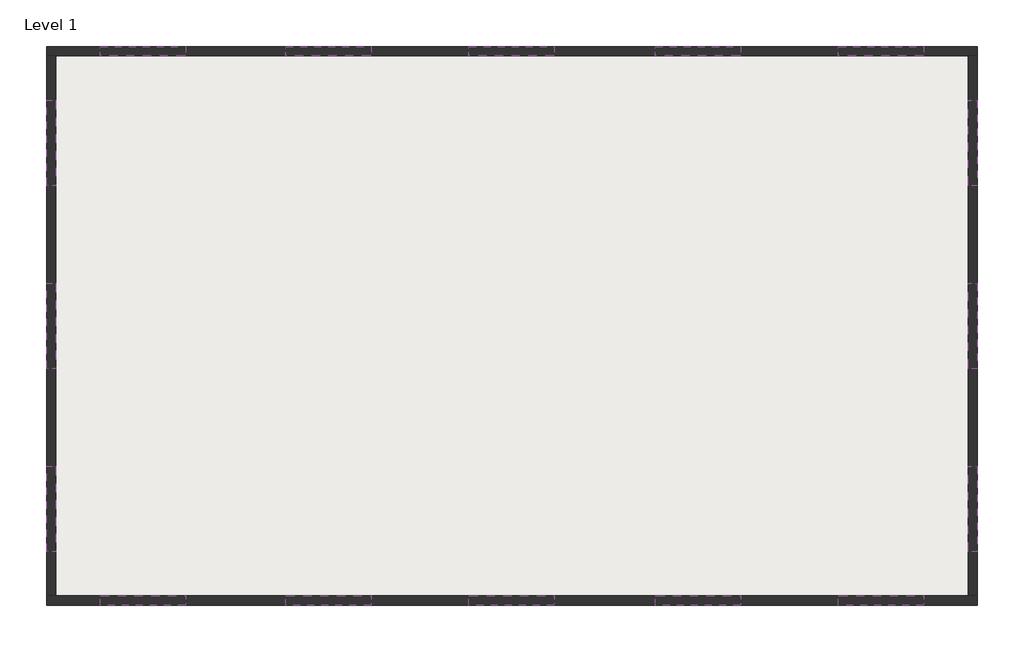
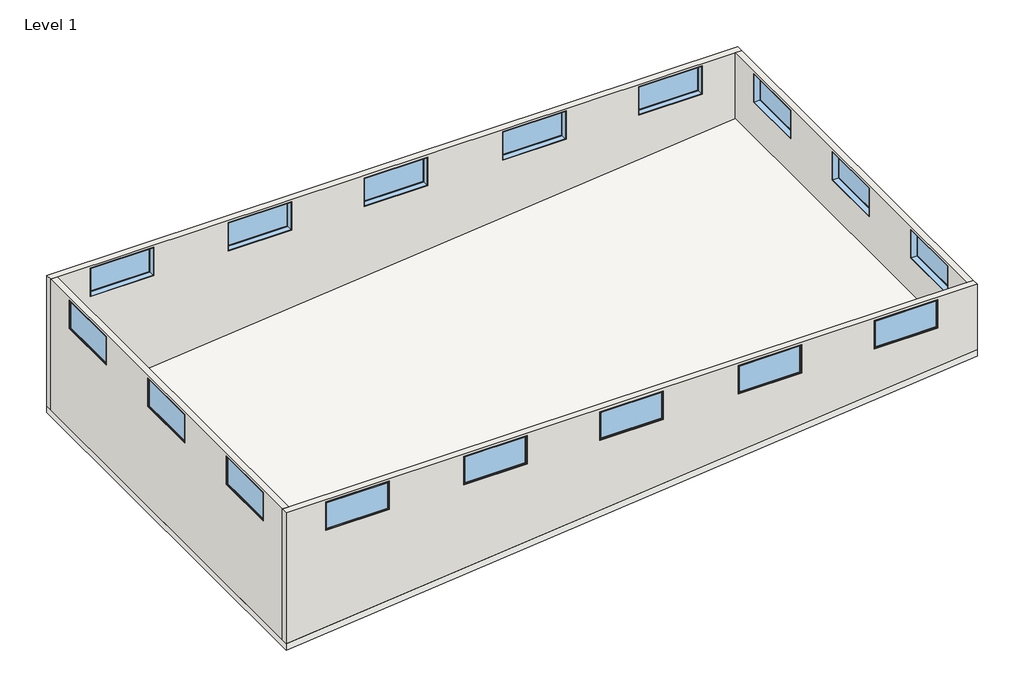
# One storey: 16 windows, 4 walls, 1 slab.
"""IFC4 building model written with IfcOpenShell, lengths in millimetres."""

import ifcopenshell
import ifcopenshell.guid

model = None  # the IFC model being written
_history = None  # IfcOwnerHistory: only IFC2X3 demands one
_inside = {}  # id of a spatial element -> (the spatial element, [elements in it])
_under = {}  # id of a project, library or spatial element -> (it, [spatial elements below it])
_declared = {}  # id of a project -> (the project, [libraries it declares])
_typed = {}  # id of a type object -> (the type object, [elements of that type])
_made_of = {}  # id of a material, layer set ... -> (it, [elements and type objects made of it])


def new_model(schema):
    """Start an empty IFC model of exactly this schema.

    Asked for "IFC4X3", IfcOpenShell would pick the latest addendum, in which some entities
    have other attributes; the version numbers below select the first issue.
    IFC2X3 requires an IfcOwnerHistory on every rooted entity: one is made here for all.
    """
    global model, _history
    if schema == "IFC4X3":
        model = ifcopenshell.file(schema_version=(4, 3, 0, 0))
    else:
        model = ifcopenshell.file(schema=schema)
    _inside.clear()
    _under.clear()
    _declared.clear()
    _typed.clear()
    _made_of.clear()
    _history = None
    if model.schema == "IFC2X3":
        org = make("IfcOrganization", Name="unknown")
        user = make(
            "IfcPersonAndOrganization",
            ThePerson=make("IfcPerson", FamilyName="unknown"),
            TheOrganization=org,
        )
        app = make(
            "IfcApplication",
            ApplicationDeveloper=org,
            Version="unknown",
            ApplicationFullName="unknown",
            ApplicationIdentifier="unknown",
        )
        _history = make(
            "IfcOwnerHistory",
            OwningUser=user,
            OwningApplication=app,
            ChangeAction="ADDED",
            CreationDate=0,
        )
    return model


def make(cls, **values):
    """One entity of the class cls with the attributes given. An attribute that is None is left unset."""
    return model.create_entity(
        cls, **{name: value for name, value in values.items() if value is not None}
    )


def rooted(cls, **values):
    """An entity with a GlobalId (a new one), such as an element, a storey or a relation."""
    return make(cls, GlobalId=ifcopenshell.guid.new(), OwnerHistory=_history, **values)


def si_unit(unit_type, name, prefix=None):
    """IfcSIUnit, for example si_unit("LENGTHUNIT", "METRE", prefix="MILLI")."""
    return make("IfcSIUnit", UnitType=unit_type, Prefix=prefix, Name=name)


def assignment(units):
    """IfcUnitAssignment: the units of a project."""
    return None if units is None else make("IfcUnitAssignment", Units=units)


def point(xyz):
    """IfcCartesianPoint."""
    return None if xyz is None else make("IfcCartesianPoint", Coordinates=xyz)


def direction(xyz):
    """IfcDirection."""
    return None if xyz is None else make("IfcDirection", DirectionRatios=xyz)


def frame(location, z_axis=None, x_axis=None):
    """IfcAxis2Placement3D, a coordinate frame: its origin and axes. An axis left out is left unset."""
    return make(
        "IfcAxis2Placement3D",
        Location=point(location),
        Axis=direction(z_axis),
        RefDirection=direction(x_axis),
    )


def origin():
    """The frame at (0, 0, 0) with its axes left unset."""
    return frame((0.0, 0.0, 0.0))


def place(relative_to, where):
    """IfcLocalPlacement: puts the frame where relative to a parent placement (None: the world)."""
    return make(
        "IfcLocalPlacement", PlacementRelTo=relative_to, RelativePlacement=where
    )


def context(
    kind, dimensions, precision=None, world=None, true_north=None, identifier=None
):
    """IfcGeometricRepresentationContext, for example the 3D "Model" context."""
    return make(
        "IfcGeometricRepresentationContext",
        ContextIdentifier=identifier,
        ContextType=kind,
        CoordinateSpaceDimension=dimensions,
        Precision=precision,
        WorldCoordinateSystem=world,
        TrueNorth=true_north,
    )


def project(units=None, contexts=None):
    """IfcProject with its units and contexts."""
    return rooted(
        "IfcProject",
        Name="project",
        RepresentationContexts=contexts,
        UnitsInContext=assignment(units),
    )


def spatial(cls, under=None, at=None, **own):
    """A site, building, storey or space (cls), placed at a placement, below another one or the project."""
    s = rooted(cls, ObjectPlacement=at, **own)
    if under is not None:
        _under.setdefault(under.id(), (under, []))[1].append(s)
    return s


def polyline(points):
    """IfcPolyline through the points."""
    return make("IfcPolyline", Points=[point(p) for p in points])


def outline(outer, holes=None, kind="AREA"):
    """IfcArbitraryClosedProfileDef: a profile drawn as a closed curve; with holes, ...WithVoids."""
    if holes is None:
        return make("IfcArbitraryClosedProfileDef", ProfileType=kind, OuterCurve=outer)
    return make(
        "IfcArbitraryProfileDefWithVoids",
        ProfileType=kind,
        OuterCurve=outer,
        InnerCurves=holes,
    )


def extrude(swept, where, along, depth):
    """IfcExtrudedAreaSolid: the profile swept, set in the frame where, extruded along a direction by depth."""
    return make(
        "IfcExtrudedAreaSolid",
        SweptArea=swept,
        Position=where,
        ExtrudedDirection=direction(along),
        Depth=depth,
    )


def faces_of(points, faces, orient=None, outer=None):
    """IfcFace entities. A face is a list of loops; a loop is a list of indices into points, from 0.

    orient and outer hold one flag for each loop. By default every Orientation is true, the
    first loop of a face is its IfcFaceOuterBound and the others are IfcFaceBound.
    """
    made = []
    for i, loops in enumerate(faces):
        bounds = []
        for j, loop in enumerate(loops):
            is_outer = j == 0 if outer is None else outer[i][j]
            bounds.append(
                make(
                    "IfcFaceOuterBound" if is_outer else "IfcFaceBound",
                    Bound=make("IfcPolyLoop", Polygon=[points[k] for k in loop]),
                    Orientation=True if orient is None else orient[i][j],
                )
            )
        made.append(make("IfcFace", Bounds=bounds))
    return made


def faceted_brep(points, faces, orient=None, outer=None, voids=None):
    """IfcFacetedBrep: a solid bounded by flat faces; with voids (closed shells), ...WithVoids."""
    shared = [point(p) for p in points]
    hull = make("IfcClosedShell", CfsFaces=faces_of(shared, faces, orient, outer))
    if voids is None:
        return make("IfcFacetedBrep", Outer=hull)
    return make(
        "IfcFacetedBrepWithVoids",
        Outer=hull,
        Voids=[
            make(cls, CfsFaces=faces_of(shared, fs, o, b)) for cls, fs, o, b in voids
        ],
    )


def shape(context_of_items, identifier, shape_type, items):
    """IfcShapeRepresentation: the items that make up one representation, for example the "Body"."""
    return make(
        "IfcShapeRepresentation",
        ContextOfItems=context_of_items,
        RepresentationIdentifier=identifier,
        RepresentationType=shape_type,
        Items=items,
    )


def source(mapping_origin, context_of_items, identifier, shape_type, items):
    """IfcRepresentationMap: a shape defined once, which mapped items show again and again."""
    return make(
        "IfcRepresentationMap",
        MappingOrigin=mapping_origin,
        MappedRepresentation=shape(context_of_items, identifier, shape_type, items),
    )


def transform(
    local_origin,
    x_axis=None,
    y_axis=None,
    z_axis=None,
    scale=None,
    scale2=None,
    scale3=None,
    uniform=True,
):
    """IfcCartesianTransformationOperator3D, or its non-uniform kind. x_axis, y_axis, z_axis: its Axis1, 2, 3."""
    if uniform:
        return make(
            "IfcCartesianTransformationOperator3D",
            Axis1=direction(x_axis),
            Axis2=direction(y_axis),
            LocalOrigin=point(local_origin),
            Scale=scale,
            Axis3=direction(z_axis),
        )
    return make(
        "IfcCartesianTransformationOperator3DnonUniform",
        Axis1=direction(x_axis),
        Axis2=direction(y_axis),
        LocalOrigin=point(local_origin),
        Scale=scale,
        Axis3=direction(z_axis),
        Scale2=scale2,
        Scale3=scale3,
    )


def mapped(mapping_source, mapping_target):
    """IfcMappedItem: shows the shape of a source again, moved by a transform."""
    return make(
        "IfcMappedItem", MappingSource=mapping_source, MappingTarget=mapping_target
    )


def made_of(thing, what):
    """Note that an element or type object is made of a material, layer set ...; save() writes the relation."""
    if what is not None:
        _made_of.setdefault(what.id(), (what, []))[1].append(thing)
    return thing


def element(
    cls,
    number,
    at=None,
    inside=None,
    cuts=None,
    type_object=None,
    material=None,
    context=None,
    identifier="Body",
    shape_type=None,
    held_by="IfcProductDefinitionShape",
    body=None,
    shapes=None,
    **own,
):
    """One element of the class cls, such as IfcWall. Its Tag is "e" and its number.

    at: its placement. inside: the storey or other place that contains it. cuts: it is an
    opening in that element (IfcRelVoidsElement). A single representation is given by context,
    identifier, shape_type and body (its items); several are given by shapes. held_by: the class
    of the entity that holds the representations. save() writes the other relations.
    """
    e = rooted(cls, Tag="e%d" % number, ObjectPlacement=at, **own)
    if body is not None:
        shapes = [shape(context, identifier, shape_type, body)]
    if shapes is not None:
        e.Representation = make(held_by, Representations=shapes)
    if inside is not None:
        _inside.setdefault(inside.id(), (inside, []))[1].append(e)
    if cuts is not None:
        rooted(
            "IfcRelVoidsElement", RelatingBuildingElement=cuts, RelatedOpeningElement=e
        )
    if type_object is not None:
        _typed.setdefault(type_object.id(), (type_object, []))[1].append(e)
    return made_of(e, material)


def aggregate(whole, parts):
    """IfcRelAggregates: a whole, such as a stair, and the parts it consists of."""
    return rooted("IfcRelAggregates", RelatingObject=whole, RelatedObjects=parts)


def save(model, path):
    """Write the relations noted so far, then the file.

    IfcRelAggregates (storeys below a building ...), IfcRelContainedInSpatialStructure (elements
    in a storey), IfcRelDefinesByType, IfcRelAssociatesMaterial and IfcRelDeclares: one each for
    every whole, place, type object, material and project.
    """
    for whole, parts in _under.values():
        aggregate(whole, parts)
    for where, things in _inside.values():
        rooted(
            "IfcRelContainedInSpatialStructure",
            RelatedElements=things,
            RelatingStructure=where,
        )
    for kind, things in _typed.values():
        rooted("IfcRelDefinesByType", RelatedObjects=things, RelatingType=kind)
    for what, things in _made_of.values():
        rooted("IfcRelAssociatesMaterial", RelatedObjects=things, RelatingMaterial=what)
    for by, libraries in _declared.values():
        rooted("IfcRelDeclares", RelatingContext=by, RelatedDefinitions=libraries)
    model.write(path)


def m_fixed_2800x_1327mm_376a1ccb(model_context):
    return source(origin(), model_context, "Body", "SweptSolid", [
        extrude(outline(polyline([(-1337.0, 130.4), (1337.0, 130.4), (1337.0, 118.4), (-1337.0, 118.4), (-1337.0, 130.4)])), frame((0.0, 0.0, 978.0), z_axis=(0.0, 0.0, 1.0), x_axis=(1.0, 0.0, 0.0)), (0.0, 0.0, 1.0), 1201.2),
        extrude(outline(polyline([(2223.2, -1381.0), (934.0, -1381.0), (934.0, 1381.0), (2223.2, 1381.0), (2223.2, -1381.0)]), holes=[polyline([(2179.2, -1337.0), (2179.2, 1337.0), (978.0, 1337.0), (978.0, -1337.0), (2179.2, -1337.0)])]), frame((0.0, 102.4, 0.0), z_axis=(0.0, 1.0, 0.0), x_axis=(0.0, 0.0, 1.0)), (0.0, 0.0, 1.0), 44.0),
        extrude(outline(polyline([(2242.2, -1400.0), (915.0, -1400.0), (915.0, 1400.0), (2242.2, 1400.0), (2242.2, -1400.0)]), holes=[polyline([(2223.2, -1381.0), (2223.2, 1381.0), (934.0, 1381.0), (934.0, -1381.0), (2223.2, -1381.0)])]), frame((0.0, 102.4, 0.0), z_axis=(0.0, 1.0, 0.0), x_axis=(0.0, 0.0, 1.0)), (0.0, 0.0, 1.0), 63.0),
        extrude(outline(polyline([(2242.2, -1400.0), (915.0, -1400.0), (915.0, 1400.0), (2242.2, 1400.0), (2242.2, -1400.0)]), holes=[polyline([(2210.2, -1368.0), (2210.2, 1368.0), (947.0, 1368.0), (947.0, -1368.0), (2210.2, -1368.0)])]), frame((0.0, -139.4, 0.0), z_axis=(0.0, 1.0, 0.0), x_axis=(0.0, 0.0, 1.0)), (0.0, 0.0, 1.0), 241.8),
    ])


def m_fixed_2800x_1327mm_95955449(model_context):
    return source(origin(), model_context, "Body", "SweptSolid", [
        extrude(outline(polyline([(-1337.0, -130.4), (-1337.0, -118.4), (1337.0, -118.4), (1337.0, -130.4), (-1337.0, -130.4)])), frame((0.0, 0.0, 978.0), z_axis=(0.0, 0.0, 1.0), x_axis=(1.0, 0.0, 0.0)), (0.0, 0.0, 1.0), 1201.2),
        extrude(outline(polyline([(2223.2, -1381.0), (934.0, -1381.0), (934.0, 1381.0), (2223.2, 1381.0), (2223.2, -1381.0)]), holes=[polyline([(2179.2, -1337.0), (2179.2, 1337.0), (978.0, 1337.0), (978.0, -1337.0), (2179.2, -1337.0)])]), frame((0.0, -146.4, 0.0), z_axis=(0.0, 1.0, 0.0), x_axis=(0.0, 0.0, 1.0)), (0.0, 0.0, 1.0), 44.0),
        extrude(outline(polyline([(2242.2, -1400.0), (915.0, -1400.0), (915.0, 1400.0), (2242.2, 1400.0), (2242.2, -1400.0)]), holes=[polyline([(2223.2, -1381.0), (2223.2, 1381.0), (934.0, 1381.0), (934.0, -1381.0), (2223.2, -1381.0)])]), frame((0.0, -165.4, 0.0), z_axis=(0.0, 1.0, 0.0), x_axis=(0.0, 0.0, 1.0)), (0.0, 0.0, 1.0), 63.0),
        extrude(outline(polyline([(2242.2, -1400.0), (915.0, -1400.0), (915.0, 1400.0), (2242.2, 1400.0), (2242.2, -1400.0)]), holes=[polyline([(2210.2, -1368.0), (2210.2, 1368.0), (947.0, 1368.0), (947.0, -1368.0), (2210.2, -1368.0)])]), frame((0.0, -102.4, 0.0), z_axis=(0.0, 1.0, 0.0), x_axis=(0.0, 0.0, 1.0)), (0.0, 0.0, 1.0), 241.8),
    ])


model = new_model("IFC4")

# Units and contexts
model_context = context("Model", 3, world=origin())
ifc_project = project(units=[si_unit("LENGTHUNIT", "METRE", prefix="MILLI")], contexts=[model_context])

# Site, building, storey
site = spatial("IfcSite", under=ifc_project)
building = spatial("IfcBuilding", under=site)
storey = spatial("IfcBuildingStorey", under=building, Name="Level 1", Elevation=0.0)

# Slab
placement = place(None, origin())
element("IfcSlab", 1, ObjectType="Generic Floor - 304.8mm", at=placement, inside=storey, context=model_context, shape_type="SweptSolid", body=[
    extrude(outline(polyline([(-3354.3202089, 1177.0035739), (-306.3202089, 31657.0035739), (0.0, 31657.0035739), (-3048.0, 1177.0035739), (-3354.3202089, 1177.0035739)])), frame((0.0, -5904.6009661, 0.0), z_axis=(0.0, 1.0, 0.0), x_axis=(0.0, 0.0, 1.0)), (0.0, 0.0, 1.0), 18288.0),
])

# Walls
element("IfcWall", 2, ObjectType="Generic - 304.8mm", at=placement, inside=storey, context=model_context, shape_type="Brep", body=[
    faceted_brep([(1177.0035739, 12078.5990339, 0.0), (1177.0035739, 12078.5990339, -3048.0), (31657.0035739, 12078.5990339, 0.0), (31657.0035739, 12078.5990339, 3048.0), (31352.2035739, 12078.5990339, 3048.0), (1481.8035739, 12078.5990339, 3048.0), (1177.0035739, 12078.5990339, 3048.0), (27104.6035739, 12078.5990339, 1618.9423249), (27104.6035739, 12078.5990339, 2946.1423249), (29904.6035739, 12078.5990339, 2946.1423249), (29904.6035739, 12078.5990339, 1618.9423249), (21104.6035739, 12078.5990339, 1618.9423249), (21104.6035739, 12078.5990339, 2946.1423249), (23904.6035739, 12078.5990339, 2946.1423249), (23904.6035739, 12078.5990339, 1618.9423249), (9004.6035739, 12078.5990339, 1618.9423249), (9004.6035739, 12078.5990339, 2946.1423249), (11804.6035739, 12078.5990339, 2946.1423249), (11804.6035739, 12078.5990339, 1618.9423249), (2929.4035739, 12078.5990339, 1618.9423249), (2929.4035739, 12078.5990339, 2946.1423249), (5729.4035739, 12078.5990339, 2946.1423249), (5729.4035739, 12078.5990339, 1618.9423249), (15004.6035739, 12078.5990339, 1595.0), (15004.6035739, 12078.5990339, 2922.2), (17804.6035739, 12078.5990339, 2922.2), (17804.6035739, 12078.5990339, 1595.0), (1177.0035739, 12383.3990339, 0.0), (1177.0035739, 12383.3990339, 3048.0), (31657.0035739, 12383.3990339, 3048.0), (31657.0035739, 12383.3990339, 0.0), (1177.0035739, 12383.3990339, -3048.0), (27104.6035739, 12383.3990339, 1618.9423249), (29904.6035739, 12383.3990339, 1618.9423249), (29904.6035739, 12383.3990339, 2946.1423249), (27104.6035739, 12383.3990339, 2946.1423249), (21104.6035739, 12383.3990339, 1618.9423249), (23904.6035739, 12383.3990339, 1618.9423249), (23904.6035739, 12383.3990339, 2946.1423249), (21104.6035739, 12383.3990339, 2946.1423249), (9004.6035739, 12383.3990339, 1618.9423249), (11804.6035739, 12383.3990339, 1618.9423249), (11804.6035739, 12383.3990339, 2946.1423249), (9004.6035739, 12383.3990339, 2946.1423249), (2929.4035739, 12383.3990339, 1618.9423249), (5729.4035739, 12383.3990339, 1618.9423249), (5729.4035739, 12383.3990339, 2946.1423249), (2929.4035739, 12383.3990339, 2946.1423249), (15004.6035739, 12383.3990339, 1595.0), (17804.6035739, 12383.3990339, 1595.0), (17804.6035739, 12383.3990339, 2922.2), (15004.6035739, 12383.3990339, 2922.2)], [[[0, 1, 2, 3, 4, 5, 6], [7, 8, 9, 10], [11, 12, 13, 14], [15, 16, 17, 18], [19, 20, 21, 22], [23, 24, 25, 26]], [[27, 28, 29, 30, 31], [32, 33, 34, 35], [36, 37, 38, 39], [40, 41, 42, 43], [44, 45, 46, 47], [48, 49, 50, 51]], [[6, 5, 4, 3, 29, 28]], [[2, 1, 31, 30]], [[3, 2, 30, 29]], [[1, 0, 6, 28, 27, 31]], [[8, 7, 32, 35]], [[9, 8, 35, 34]], [[10, 9, 34, 33]], [[7, 10, 33, 32]], [[12, 11, 36, 39]], [[13, 12, 39, 38]], [[14, 13, 38, 37]], [[11, 14, 37, 36]], [[16, 15, 40, 43]], [[17, 16, 43, 42]], [[18, 17, 42, 41]], [[15, 18, 41, 40]], [[20, 19, 44, 47]], [[21, 20, 47, 46]], [[22, 21, 46, 45]], [[19, 22, 45, 44]], [[24, 23, 48, 51]], [[25, 24, 51, 50]], [[26, 25, 50, 49]], [[23, 26, 49, 48]]]),
])
element("IfcWall", 3, ObjectType="Generic - 304.8mm", at=placement, inside=storey, context=model_context, shape_type="Brep", body=[
    faceted_brep([(31657.0035739, -5599.8009661, 0.0), (1177.0035739, -5599.8009661, -3048.0), (1177.0035739, -5599.8009661, 0.0), (1177.0035739, -5599.8009661, 3048.0), (1481.8035739, -5599.8009661, 3048.0), (31352.2035739, -5599.8009661, 3048.0), (31657.0035739, -5599.8009661, 3048.0), (15004.6035739, -5599.8009661, 1595.0), (17804.6035739, -5599.8009661, 1595.0), (17804.6035739, -5599.8009661, 2922.2), (15004.6035739, -5599.8009661, 2922.2), (2929.4035739, -5599.8009661, 1618.9423249), (5729.4035739, -5599.8009661, 1618.9423249), (5729.4035739, -5599.8009661, 2946.1423249), (2929.4035739, -5599.8009661, 2946.1423249), (9004.6035739, -5599.8009661, 1618.9423249), (11804.6035739, -5599.8009661, 1618.9423249), (11804.6035739, -5599.8009661, 2946.1423249), (9004.6035739, -5599.8009661, 2946.1423249), (21104.6035739, -5599.8009661, 1618.9423249), (23904.6035739, -5599.8009661, 1618.9423249), (23904.6035739, -5599.8009661, 2946.1423249), (21104.6035739, -5599.8009661, 2946.1423249), (27104.6035739, -5599.8009661, 1618.9423249), (29904.6035739, -5599.8009661, 1618.9423249), (29904.6035739, -5599.8009661, 2946.1423249), (27104.6035739, -5599.8009661, 2946.1423249), (31657.0035739, -5904.6009661, 0.0), (31657.0035739, -5904.6009661, 3048.0), (1177.0035739, -5904.6009661, 3048.0), (1177.0035739, -5904.6009661, 0.0), (1177.0035739, -5904.6009661, -3048.0), (15004.6035739, -5904.6009661, 1595.0), (15004.6035739, -5904.6009661, 2922.2), (17804.6035739, -5904.6009661, 2922.2), (17804.6035739, -5904.6009661, 1595.0), (2929.4035739, -5904.6009661, 1618.9423249), (2929.4035739, -5904.6009661, 2946.1423249), (5729.4035739, -5904.6009661, 2946.1423249), (5729.4035739, -5904.6009661, 1618.9423249), (9004.6035739, -5904.6009661, 1618.9423249), (9004.6035739, -5904.6009661, 2946.1423249), (11804.6035739, -5904.6009661, 2946.1423249), (11804.6035739, -5904.6009661, 1618.9423249), (21104.6035739, -5904.6009661, 1618.9423249), (21104.6035739, -5904.6009661, 2946.1423249), (23904.6035739, -5904.6009661, 2946.1423249), (23904.6035739, -5904.6009661, 1618.9423249), (27104.6035739, -5904.6009661, 1618.9423249), (27104.6035739, -5904.6009661, 2946.1423249), (29904.6035739, -5904.6009661, 2946.1423249), (29904.6035739, -5904.6009661, 1618.9423249)], [[[0, 1, 2, 3, 4, 5, 6], [7, 8, 9, 10], [11, 12, 13, 14], [15, 16, 17, 18], [19, 20, 21, 22], [23, 24, 25, 26]], [[27, 28, 29, 30, 31], [32, 33, 34, 35], [36, 37, 38, 39], [40, 41, 42, 43], [44, 45, 46, 47], [48, 49, 50, 51]], [[6, 5, 4, 3, 29, 28]], [[0, 6, 28, 27]], [[2, 1, 31, 30, 29, 3]], [[1, 0, 27, 31]], [[33, 32, 7, 10]], [[34, 33, 10, 9]], [[35, 34, 9, 8]], [[32, 35, 8, 7]], [[37, 36, 11, 14]], [[38, 37, 14, 13]], [[39, 38, 13, 12]], [[36, 39, 12, 11]], [[41, 40, 15, 18]], [[42, 41, 18, 17]], [[43, 42, 17, 16]], [[40, 43, 16, 15]], [[45, 44, 19, 22]], [[46, 45, 22, 21]], [[47, 46, 21, 20]], [[44, 47, 20, 19]], [[49, 48, 23, 26]], [[50, 49, 26, 25]], [[51, 50, 25, 24]], [[48, 51, 24, 23]]]),
])
element("IfcWall", 4, ObjectType="Generic - 304.8mm", at=placement, inside=storey, context=model_context, shape_type="Brep", body=[
    faceted_brep([(31352.2035739, 12078.5990339, 44.3356751), (31352.2035739, 12078.5990339, 0.0), (31352.2035739, -5599.8009661, 0.0), (31352.2035739, -5599.8009661, 44.3356751), (31352.2035739, -5599.8009661, 3048.0), (31352.2035739, 12078.5990339, 3048.0), (31352.2035739, -4152.2009661, 1618.9), (31352.2035739, -1352.2009661, 1618.9), (31352.2035739, -1352.2009661, 2946.1), (31352.2035739, -4152.2009661, 2946.1), (31352.2035739, 7830.9990339, 1618.9), (31352.2035739, 10630.9990339, 1618.9), (31352.2035739, 10630.9990339, 2946.1), (31352.2035739, 7830.9990339, 2946.1), (31352.2035739, 1839.3990339, 1618.9), (31352.2035739, 4639.3990339, 1618.9), (31352.2035739, 4639.3990339, 2946.1), (31352.2035739, 1839.3990339, 2946.1), (31657.0035739, 12078.5990339, 44.3356751), (31657.0035739, 12078.5990339, 3048.0), (31657.0035739, -5599.8009661, 3048.0), (31657.0035739, -5599.8009661, 44.3356751), (31657.0035739, -5599.8009661, 0.0), (31657.0035739, 12078.5990339, 0.0), (31657.0035739, -4152.2009661, 1618.9), (31657.0035739, -4152.2009661, 2946.1), (31657.0035739, -1352.2009661, 2946.1), (31657.0035739, -1352.2009661, 1618.9), (31657.0035739, 7830.9990339, 1618.9), (31657.0035739, 7830.9990339, 2946.1), (31657.0035739, 10630.9990339, 2946.1), (31657.0035739, 10630.9990339, 1618.9), (31657.0035739, 1839.3990339, 1618.9), (31657.0035739, 1839.3990339, 2946.1), (31657.0035739, 4639.3990339, 2946.1), (31657.0035739, 4639.3990339, 1618.9)], [[[0, 1, 2, 3, 4, 5], [6, 7, 8, 9], [10, 11, 12, 13], [14, 15, 16, 17]], [[18, 19, 20, 21, 22, 23], [24, 25, 26, 27], [28, 29, 30, 31], [32, 33, 34, 35]], [[5, 4, 20, 19]], [[2, 1, 23, 22]], [[1, 0, 5, 19, 18, 23]], [[3, 2, 22, 21, 20, 4]], [[25, 24, 6, 9]], [[26, 25, 9, 8]], [[27, 26, 8, 7]], [[24, 27, 7, 6]], [[29, 28, 10, 13]], [[30, 29, 13, 12]], [[31, 30, 12, 11]], [[28, 31, 11, 10]], [[33, 32, 14, 17]], [[34, 33, 17, 16]], [[35, 34, 16, 15]], [[32, 35, 15, 14]]]),
])
element("IfcWall", 5, ObjectType="Generic - 304.8mm", at=placement, inside=storey, context=model_context, shape_type="SweptSolid", body=[
    extrude(outline(polyline([(12078.5990339, -3048.0), (-5599.8009661, -3048.0), (-5599.8009661, 3048.0), (12078.5990339, 3048.0), (12078.5990339, -3048.0)]), holes=[polyline([(1839.3990339, 2946.1), (1839.3990339, 1618.9), (4639.3990339, 1618.9), (4639.3990339, 2946.1), (1839.3990339, 2946.1)]), polyline([(-4152.2009661, 2946.1), (-4152.2009661, 1618.9), (-1352.2009661, 1618.9), (-1352.2009661, 2946.1), (-4152.2009661, 2946.1)]), polyline([(7830.9990339, 2946.1), (7830.9990339, 1618.9), (10630.9990339, 1618.9), (10630.9990339, 2946.1), (7830.9990339, 2946.1)])]), frame((1177.0035739, 0.0, 0.0), z_axis=(1.0, 0.0, 0.0), x_axis=(0.0, 1.0, 0.0)), (0.0, 0.0, 1.0), 304.8),
])

# Windows
m_fixed_2800x_1327mm_shape = m_fixed_2800x_1327mm_376a1ccb(model_context)
element("IfcWindow", 6, ObjectType="M_Fixed : 2800x 1327mm", at=placement, inside=storey, context=model_context, shape_type="MappedRepresentation", body=[
    mapped(m_fixed_2800x_1327mm_shape, transform((28504.6035739, 12217.9990339, 703.9423249), x_axis=(1.0, 0.0, 0.0), y_axis=(0.0, 1.0, 0.0), z_axis=(0.0, 0.0, 1.0))),
])
element("IfcWindow", 7, ObjectType="M_Fixed : 2800x 1327mm", at=placement, inside=storey, context=model_context, shape_type="MappedRepresentation", body=[
    mapped(m_fixed_2800x_1327mm_shape, transform((22504.6035739, 12217.9990339, 703.9423249), x_axis=(1.0, 0.0, 0.0), y_axis=(0.0, 1.0, 0.0), z_axis=(0.0, 0.0, 1.0))),
])
element("IfcWindow", 8, ObjectType="M_Fixed : 2800x 1327mm", at=placement, inside=storey, context=model_context, shape_type="MappedRepresentation", body=[
    mapped(m_fixed_2800x_1327mm_shape, transform((10404.6035739, 12217.9990339, 703.9423249), x_axis=(1.0, 0.0, 0.0), y_axis=(0.0, 1.0, 0.0), z_axis=(0.0, 0.0, 1.0))),
])
element("IfcWindow", 9, ObjectType="M_Fixed : 2800x 1327mm", at=placement, inside=storey, context=model_context, shape_type="MappedRepresentation", body=[
    mapped(m_fixed_2800x_1327mm_shape, transform((4329.4035739, 12217.9990339, 703.9423249), x_axis=(1.0, 0.0, 0.0), y_axis=(0.0, 1.0, 0.0), z_axis=(0.0, 0.0, 1.0))),
])
element("IfcWindow", 10, ObjectType="M_Fixed : 2800x 1327mm", at=placement, inside=storey, context=model_context, shape_type="MappedRepresentation", body=[
    mapped(m_fixed_2800x_1327mm_shape, transform((16404.6035739, 12217.9990339, 680.0), x_axis=(1.0, 0.0, 0.0), y_axis=(0.0, 1.0, 0.0), z_axis=(0.0, 0.0, 1.0))),
])
element("IfcWindow", 11, ObjectType="M_Fixed : 2800x 1327mm", at=placement, inside=storey, context=model_context, shape_type="MappedRepresentation", body=[
    mapped(m_fixed_2800x_1327mm_shape, transform((1342.4035739, 3239.3990339, 703.9), x_axis=(0.0, 1.0, 0.0), y_axis=(-1.0, 0.0, 0.0), z_axis=(0.0, 0.0, 1.0))),
])
element("IfcWindow", 12, ObjectType="M_Fixed : 2800x 1327mm", at=placement, inside=storey, context=model_context, shape_type="MappedRepresentation", body=[
    mapped(m_fixed_2800x_1327mm_shape, transform((1342.4035739, 9230.9990339, 703.9), x_axis=(0.0, 1.0, 0.0), y_axis=(-1.0, 0.0, 0.0), z_axis=(0.0, 0.0, 1.0))),
])
element("IfcWindow", 13, ObjectType="M_Fixed : 2800x 1327mm", at=placement, inside=storey, context=model_context, shape_type="MappedRepresentation", body=[
    mapped(m_fixed_2800x_1327mm_shape, transform((1342.4035739, -2752.2009661, 703.9), x_axis=(0.0, 1.0, 0.0), y_axis=(-1.0, 0.0, 0.0), z_axis=(0.0, 0.0, 1.0))),
])
m_fixed_2800x_1327mm_2_shape = m_fixed_2800x_1327mm_95955449(model_context)
element("IfcWindow", 14, ObjectType="M_Fixed : 2800x 1327mm", at=placement, inside=storey, context=model_context, shape_type="MappedRepresentation", body=[
    mapped(m_fixed_2800x_1327mm_2_shape, transform((28504.6035739, -5739.2009661, 703.9423249), x_axis=(1.0, 0.0, 0.0), y_axis=(0.0, 1.0, 0.0), z_axis=(0.0, 0.0, 1.0))),
])
element("IfcWindow", 15, ObjectType="M_Fixed : 2800x 1327mm", at=placement, inside=storey, context=model_context, shape_type="MappedRepresentation", body=[
    mapped(m_fixed_2800x_1327mm_2_shape, transform((22504.6035739, -5739.2009661, 703.9423249), x_axis=(1.0, 0.0, 0.0), y_axis=(0.0, 1.0, 0.0), z_axis=(0.0, 0.0, 1.0))),
])
element("IfcWindow", 16, ObjectType="M_Fixed : 2800x 1327mm", at=placement, inside=storey, context=model_context, shape_type="MappedRepresentation", body=[
    mapped(m_fixed_2800x_1327mm_2_shape, transform((10404.6035739, -5739.2009661, 703.9423249), x_axis=(1.0, 0.0, 0.0), y_axis=(0.0, 1.0, 0.0), z_axis=(0.0, 0.0, 1.0))),
])
element("IfcWindow", 17, ObjectType="M_Fixed : 2800x 1327mm", at=placement, inside=storey, context=model_context, shape_type="MappedRepresentation", body=[
    mapped(m_fixed_2800x_1327mm_2_shape, transform((4329.4035739, -5739.2009661, 703.9423249), x_axis=(1.0, 0.0, 0.0), y_axis=(0.0, 1.0, 0.0), z_axis=(0.0, 0.0, 1.0))),
])
element("IfcWindow", 18, ObjectType="M_Fixed : 2800x 1327mm", at=placement, inside=storey, context=model_context, shape_type="MappedRepresentation", body=[
    mapped(m_fixed_2800x_1327mm_2_shape, transform((16404.6035739, -5739.2009661, 680.0), x_axis=(1.0, 0.0, 0.0), y_axis=(0.0, 1.0, 0.0), z_axis=(0.0, 0.0, 1.0))),
])
element("IfcWindow", 19, ObjectType="M_Fixed : 2800x 1327mm", at=placement, inside=storey, context=model_context, shape_type="MappedRepresentation", body=[
    mapped(m_fixed_2800x_1327mm_2_shape, transform((31491.6035739, 3239.3990339, 703.9), x_axis=(0.0, 1.0, 0.0), y_axis=(-1.0, 0.0, 0.0), z_axis=(0.0, 0.0, 1.0))),
])
element("IfcWindow", 20, ObjectType="M_Fixed : 2800x 1327mm", at=placement, inside=storey, context=model_context, shape_type="MappedRepresentation", body=[
    mapped(m_fixed_2800x_1327mm_2_shape, transform((31491.6035739, 9230.9990339, 703.9), x_axis=(0.0, 1.0, 0.0), y_axis=(-1.0, 0.0, 0.0), z_axis=(0.0, 0.0, 1.0))),
])
element("IfcWindow", 21, ObjectType="M_Fixed : 2800x 1327mm", at=placement, inside=storey, context=model_context, shape_type="MappedRepresentation", body=[
    mapped(m_fixed_2800x_1327mm_2_shape, transform((31491.6035739, -2752.2009661, 703.9), x_axis=(0.0, 1.0, 0.0), y_axis=(-1.0, 0.0, 0.0), z_axis=(0.0, 0.0, 1.0))),
])

save(model, "model.ifc")

# Revit data of these elements
# Project information
#   Project Issue Date = "Issue Date"
#   Project Status = "Project Status"
#   Client Name = "Owner"
#   Project Address = "Enter address here"
#   Project Name = "Project Name"
#   Project Number = "Project Number"
# Type "Generic Floor - 304.8mm"
#   Function = 0
#   Layers, outside or top first: 304.8 mm no material (function 1)
# Type "Generic - 304.8mm"
#   Layers, outside or top first: 304.8 mm no material (function 1)
# Type "M_Fixed : 2800x 1327mm"
#   Type Mark = "46"
#   Height = 1327.2 mm
#   Default Sill Height = 915 mm
#   Width = 2800 mm
#   Window Inset = 19 mm
#   Frame Exterior Material = Sash
#   Frame Interior Material = Sash
#   Glass Pane Material = Glass
#   Sash = Sash
#   Wall Closure = (empty or 0)
# Element 1 (IfcSlab, "Generic Floor - 304.8mm")
#   Height Offset From Level = -3048 mm
#   Phase Created = New Construction
#   Materials on its faces: "Default Floor"
# Elements 2, 3 (IfcWall, "Generic - 304.8mm")
#   Top Offset = 0 mm
#   Base Offset = 0 mm
#   wall height = 3048 mm
#   Phase Created = New Construction
#   Base Constraint = Level 1
#   Top Constraint = Level 2
#   Materials on its faces: "Default Wall"
# Element 4 (IfcWall, "Generic - 304.8mm")
#   built-in parameter 1001111 = 44.336 mm
#   Top Offset = 0 mm
#   Base Offset = 44.336 mm
#   Unconnected Height = 3003.664 mm
#   wall height = 3003.664 mm
#   Phase Created = New Construction
#   Base Constraint = Level 1
#   Materials on its faces: "Default Wall"
# Element 5 (IfcWall, "Generic - 304.8mm")
#   built-in parameter 1001111 = -3048 mm
#   Top Offset = 0 mm
#   Base Offset = -3048 mm
#   Unconnected Height = 6096 mm
#   wall height = 6096 mm
#   Phase Created = New Construction
#   Base Constraint = Level 1
#   Materials on its faces: "Default Wall"
# Element 6 (IfcWindow, "M_Fixed : 2800x 1327mm")
#   Mark = "38"
#   Phase Created = New Construction
#   Materials on its faces: "Sash", "Glass"
# Element 7 (IfcWindow, "M_Fixed : 2800x 1327mm")
#   Mark = "39"
#   Phase Created = New Construction
#   Materials on its faces: "Sash", "Glass"
# Element 8 (IfcWindow, "M_Fixed : 2800x 1327mm")
#   Mark = "41"
#   Phase Created = New Construction
#   Materials on its faces: "Sash", "Glass"
# Element 9 (IfcWindow, "M_Fixed : 2800x 1327mm")
#   Mark = "42"
#   Phase Created = New Construction
#   Materials on its faces: "Sash", "Glass"
# Element 10 (IfcWindow, "M_Fixed : 2800x 1327mm")
#   Mark = "43"
#   Phase Created = New Construction
#   Materials on its faces: "Sash", "Glass"
# Element 11 (IfcWindow, "M_Fixed : 2800x 1327mm")
#   Mark = "69"
#   Phase Created = New Construction
#   Materials on its faces: "Sash", "Glass"
# Element 12 (IfcWindow, "M_Fixed : 2800x 1327mm")
#   Mark = "70"
#   Phase Created = New Construction
#   Materials on its faces: "Sash", "Glass"
# Element 13 (IfcWindow, "M_Fixed : 2800x 1327mm")
#   Mark = "71"
#   Phase Created = New Construction
#   Materials on its faces: "Sash", "Glass"
# Element 14 (IfcWindow, "M_Fixed : 2800x 1327mm")
#   Mark = "54"
#   Phase Created = New Construction
#   Materials on its faces: "Sash", "Glass"
# Element 15 (IfcWindow, "M_Fixed : 2800x 1327mm")
#   Mark = "55"
#   Phase Created = New Construction
#   Materials on its faces: "Sash", "Glass"
# Element 16 (IfcWindow, "M_Fixed : 2800x 1327mm")
#   Mark = "56"
#   Phase Created = New Construction
#   Materials on its faces: "Sash", "Glass"
# Element 17 (IfcWindow, "M_Fixed : 2800x 1327mm")
#   Mark = "57"
#   Phase Created = New Construction
#   Materials on its faces: "Sash", "Glass"
# Element 18 (IfcWindow, "M_Fixed : 2800x 1327mm")
#   Mark = "58"
#   Phase Created = New Construction
#   Materials on its faces: "Sash", "Glass"
# Element 19 (IfcWindow, "M_Fixed : 2800x 1327mm")
#   Mark = "78"
#   Phase Created = New Construction
#   Materials on its faces: "Sash", "Glass"
# Element 20 (IfcWindow, "M_Fixed : 2800x 1327mm")
#   Mark = "79"
#   Phase Created = New Construction
#   Materials on its faces: "Sash", "Glass"
# Element 21 (IfcWindow, "M_Fixed : 2800x 1327mm")
#   Mark = "80"
#   Phase Created = New Construction
#   Materials on its faces: "Sash", "Glass"
# Materials
#   "Sash": class "Wood", colour RGB 136 99 55, transparency 0
#   "Glass": class "Glass", colour RGB 0 128 192, transparency 0.9, Description = "Soda Lime Glass", Cost = 0
#   "Default Floor": class "Miscellaneous", colour RGB 127 127 127, transparency 0, Cost = 0
#   "Default Wall": class "Miscellaneous", colour RGB 128 128 128, transparency 0, Cost = 0
# Room at (16404.883, 3376.313) mm, phase "New Construction", upper level "Level 2", upper offset 0 mm, lower offset -3048 mm
#   Number = "1"
#   Name = "Room"
